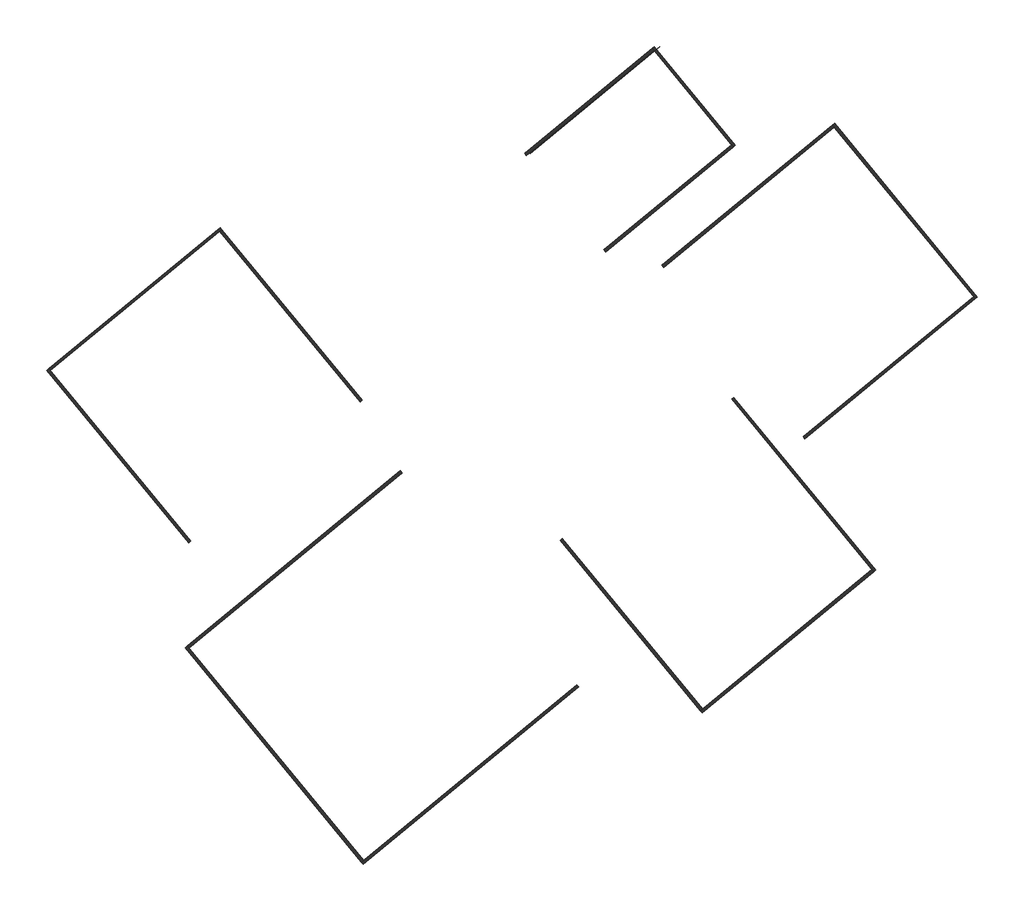
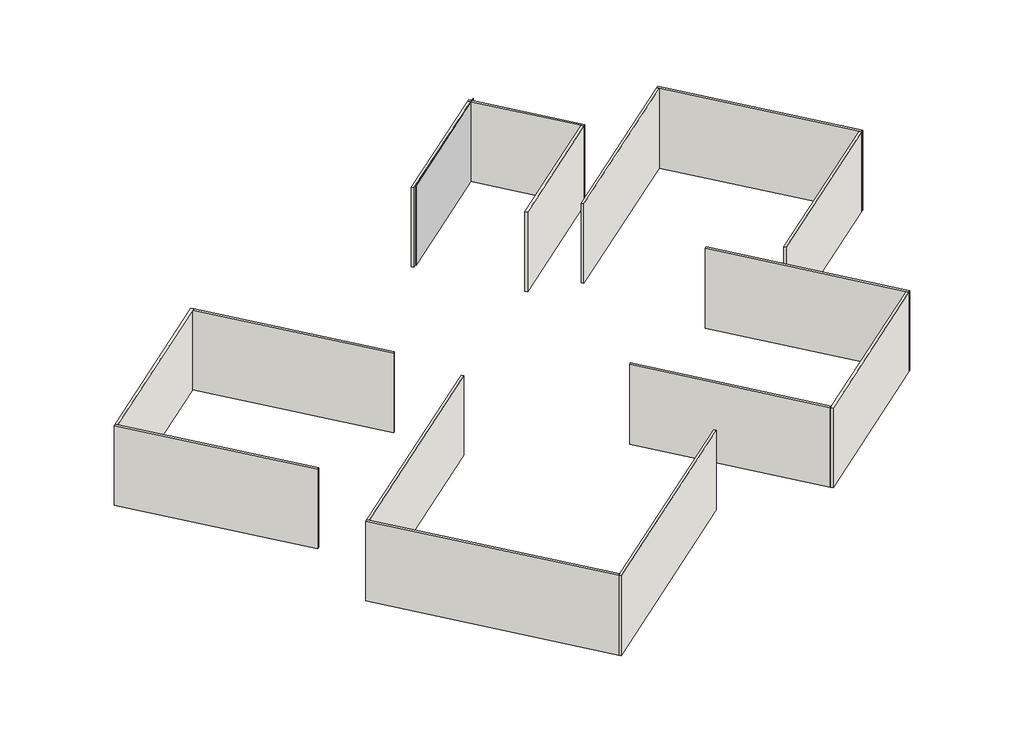
# One storey: 15 walls, 1 plate.
"""IFC4 building model written with IfcOpenShell, lengths in millimetres."""

import ifcopenshell
import ifcopenshell.guid

model = None  # the IFC model being written
_history = None  # IfcOwnerHistory: only IFC2X3 demands one
_inside = {}  # id of a spatial element -> (the spatial element, [elements in it])
_under = {}  # id of a project, library or spatial element -> (it, [spatial elements below it])
_declared = {}  # id of a project -> (the project, [libraries it declares])
_typed = {}  # id of a type object -> (the type object, [elements of that type])
_made_of = {}  # id of a material, layer set ... -> (it, [elements and type objects made of it])


def new_model(schema):
    """Start an empty IFC model of exactly this schema.

    Asked for "IFC4X3", IfcOpenShell would pick the latest addendum, in which some entities
    have other attributes; the version numbers below select the first issue.
    IFC2X3 requires an IfcOwnerHistory on every rooted entity: one is made here for all.
    """
    global model, _history
    if schema == "IFC4X3":
        model = ifcopenshell.file(schema_version=(4, 3, 0, 0))
    else:
        model = ifcopenshell.file(schema=schema)
    _inside.clear()
    _under.clear()
    _declared.clear()
    _typed.clear()
    _made_of.clear()
    _history = None
    if model.schema == "IFC2X3":
        org = make("IfcOrganization", Name="unknown")
        user = make(
            "IfcPersonAndOrganization",
            ThePerson=make("IfcPerson", FamilyName="unknown"),
            TheOrganization=org,
        )
        app = make(
            "IfcApplication",
            ApplicationDeveloper=org,
            Version="unknown",
            ApplicationFullName="unknown",
            ApplicationIdentifier="unknown",
        )
        _history = make(
            "IfcOwnerHistory",
            OwningUser=user,
            OwningApplication=app,
            ChangeAction="ADDED",
            CreationDate=0,
        )
    return model


def make(cls, **values):
    """One entity of the class cls with the attributes given. An attribute that is None is left unset."""
    return model.create_entity(
        cls, **{name: value for name, value in values.items() if value is not None}
    )


def rooted(cls, **values):
    """An entity with a GlobalId (a new one), such as an element, a storey or a relation."""
    return make(cls, GlobalId=ifcopenshell.guid.new(), OwnerHistory=_history, **values)


def si_unit(unit_type, name, prefix=None):
    """IfcSIUnit, for example si_unit("LENGTHUNIT", "METRE", prefix="MILLI")."""
    return make("IfcSIUnit", UnitType=unit_type, Prefix=prefix, Name=name)


def assignment(units):
    """IfcUnitAssignment: the units of a project."""
    return None if units is None else make("IfcUnitAssignment", Units=units)


def point(xyz):
    """IfcCartesianPoint."""
    return None if xyz is None else make("IfcCartesianPoint", Coordinates=xyz)


def direction(xyz):
    """IfcDirection."""
    return None if xyz is None else make("IfcDirection", DirectionRatios=xyz)


def frame(location, z_axis=None, x_axis=None):
    """IfcAxis2Placement3D, a coordinate frame: its origin and axes. An axis left out is left unset."""
    return make(
        "IfcAxis2Placement3D",
        Location=point(location),
        Axis=direction(z_axis),
        RefDirection=direction(x_axis),
    )


def origin():
    """The frame at (0, 0, 0) with its axes left unset."""
    return frame((0.0, 0.0, 0.0))


def origin_with_axes():
    """The frame at (0, 0, 0) with the z axis (0, 0, 1) and the x axis (1, 0, 0) written out."""
    return frame((0.0, 0.0, 0.0), z_axis=(0.0, 0.0, 1.0), x_axis=(1.0, 0.0, 0.0))


def place(relative_to, where):
    """IfcLocalPlacement: puts the frame where relative to a parent placement (None: the world)."""
    return make(
        "IfcLocalPlacement", PlacementRelTo=relative_to, RelativePlacement=where
    )


def context(
    kind, dimensions, precision=None, world=None, true_north=None, identifier=None
):
    """IfcGeometricRepresentationContext, for example the 3D "Model" context."""
    return make(
        "IfcGeometricRepresentationContext",
        ContextIdentifier=identifier,
        ContextType=kind,
        CoordinateSpaceDimension=dimensions,
        Precision=precision,
        WorldCoordinateSystem=world,
        TrueNorth=true_north,
    )


def project(units=None, contexts=None):
    """IfcProject with its units and contexts."""
    return rooted(
        "IfcProject",
        Name="project",
        RepresentationContexts=contexts,
        UnitsInContext=assignment(units),
    )


def spatial(cls, under=None, at=None, **own):
    """A site, building, storey or space (cls), placed at a placement, below another one or the project."""
    s = rooted(cls, ObjectPlacement=at, **own)
    if under is not None:
        _under.setdefault(under.id(), (under, []))[1].append(s)
    return s


def polyline(points):
    """IfcPolyline through the points."""
    return make("IfcPolyline", Points=[point(p) for p in points])


def outline(outer, holes=None, kind="AREA"):
    """IfcArbitraryClosedProfileDef: a profile drawn as a closed curve; with holes, ...WithVoids."""
    if holes is None:
        return make("IfcArbitraryClosedProfileDef", ProfileType=kind, OuterCurve=outer)
    return make(
        "IfcArbitraryProfileDefWithVoids",
        ProfileType=kind,
        OuterCurve=outer,
        InnerCurves=holes,
    )


def extrude(swept, where, along, depth):
    """IfcExtrudedAreaSolid: the profile swept, set in the frame where, extruded along a direction by depth."""
    return make(
        "IfcExtrudedAreaSolid",
        SweptArea=swept,
        Position=where,
        ExtrudedDirection=direction(along),
        Depth=depth,
    )


def faces_of(points, faces, orient=None, outer=None):
    """IfcFace entities. A face is a list of loops; a loop is a list of indices into points, from 0.

    orient and outer hold one flag for each loop. By default every Orientation is true, the
    first loop of a face is its IfcFaceOuterBound and the others are IfcFaceBound.
    """
    made = []
    for i, loops in enumerate(faces):
        bounds = []
        for j, loop in enumerate(loops):
            is_outer = j == 0 if outer is None else outer[i][j]
            bounds.append(
                make(
                    "IfcFaceOuterBound" if is_outer else "IfcFaceBound",
                    Bound=make("IfcPolyLoop", Polygon=[points[k] for k in loop]),
                    Orientation=True if orient is None else orient[i][j],
                )
            )
        made.append(make("IfcFace", Bounds=bounds))
    return made


def faceted_brep(points, faces, orient=None, outer=None, voids=None):
    """IfcFacetedBrep: a solid bounded by flat faces; with voids (closed shells), ...WithVoids."""
    shared = [point(p) for p in points]
    hull = make("IfcClosedShell", CfsFaces=faces_of(shared, faces, orient, outer))
    if voids is None:
        return make("IfcFacetedBrep", Outer=hull)
    return make(
        "IfcFacetedBrepWithVoids",
        Outer=hull,
        Voids=[
            make(cls, CfsFaces=faces_of(shared, fs, o, b)) for cls, fs, o, b in voids
        ],
    )


def shape(context_of_items, identifier, shape_type, items):
    """IfcShapeRepresentation: the items that make up one representation, for example the "Body"."""
    return make(
        "IfcShapeRepresentation",
        ContextOfItems=context_of_items,
        RepresentationIdentifier=identifier,
        RepresentationType=shape_type,
        Items=items,
    )


def source(mapping_origin, context_of_items, identifier, shape_type, items):
    """IfcRepresentationMap: a shape defined once, which mapped items show again and again."""
    return make(
        "IfcRepresentationMap",
        MappingOrigin=mapping_origin,
        MappedRepresentation=shape(context_of_items, identifier, shape_type, items),
    )


def transform(
    local_origin,
    x_axis=None,
    y_axis=None,
    z_axis=None,
    scale=None,
    scale2=None,
    scale3=None,
    uniform=True,
):
    """IfcCartesianTransformationOperator3D, or its non-uniform kind. x_axis, y_axis, z_axis: its Axis1, 2, 3."""
    if uniform:
        return make(
            "IfcCartesianTransformationOperator3D",
            Axis1=direction(x_axis),
            Axis2=direction(y_axis),
            LocalOrigin=point(local_origin),
            Scale=scale,
            Axis3=direction(z_axis),
        )
    return make(
        "IfcCartesianTransformationOperator3DnonUniform",
        Axis1=direction(x_axis),
        Axis2=direction(y_axis),
        LocalOrigin=point(local_origin),
        Scale=scale,
        Axis3=direction(z_axis),
        Scale2=scale2,
        Scale3=scale3,
    )


def mapped(mapping_source, mapping_target):
    """IfcMappedItem: shows the shape of a source again, moved by a transform."""
    return make(
        "IfcMappedItem", MappingSource=mapping_source, MappingTarget=mapping_target
    )


def made_of(thing, what):
    """Note that an element or type object is made of a material, layer set ...; save() writes the relation."""
    if what is not None:
        _made_of.setdefault(what.id(), (what, []))[1].append(thing)
    return thing


def element(
    cls,
    number,
    at=None,
    inside=None,
    cuts=None,
    type_object=None,
    material=None,
    context=None,
    identifier="Body",
    shape_type=None,
    held_by="IfcProductDefinitionShape",
    body=None,
    shapes=None,
    **own,
):
    """One element of the class cls, such as IfcWall. Its Tag is "e" and its number.

    at: its placement. inside: the storey or other place that contains it. cuts: it is an
    opening in that element (IfcRelVoidsElement). A single representation is given by context,
    identifier, shape_type and body (its items); several are given by shapes. held_by: the class
    of the entity that holds the representations. save() writes the other relations.
    """
    e = rooted(cls, Tag="e%d" % number, ObjectPlacement=at, **own)
    if body is not None:
        shapes = [shape(context, identifier, shape_type, body)]
    if shapes is not None:
        e.Representation = make(held_by, Representations=shapes)
    if inside is not None:
        _inside.setdefault(inside.id(), (inside, []))[1].append(e)
    if cuts is not None:
        rooted(
            "IfcRelVoidsElement", RelatingBuildingElement=cuts, RelatedOpeningElement=e
        )
    if type_object is not None:
        _typed.setdefault(type_object.id(), (type_object, []))[1].append(e)
    return made_of(e, material)


def aggregate(whole, parts):
    """IfcRelAggregates: a whole, such as a stair, and the parts it consists of."""
    return rooted("IfcRelAggregates", RelatingObject=whole, RelatedObjects=parts)


def save(model, path):
    """Write the relations noted so far, then the file.

    IfcRelAggregates (storeys below a building ...), IfcRelContainedInSpatialStructure (elements
    in a storey), IfcRelDefinesByType, IfcRelAssociatesMaterial and IfcRelDeclares: one each for
    every whole, place, type object, material and project.
    """
    for whole, parts in _under.values():
        aggregate(whole, parts)
    for where, things in _inside.values():
        rooted(
            "IfcRelContainedInSpatialStructure",
            RelatedElements=things,
            RelatingStructure=where,
        )
    for kind, things in _typed.values():
        rooted("IfcRelDefinesByType", RelatedObjects=things, RelatingType=kind)
    for what, things in _made_of.values():
        rooted("IfcRelAssociatesMaterial", RelatedObjects=things, RelatingMaterial=what)
    for by, libraries in _declared.values():
        rooted("IfcRelDeclares", RelatingContext=by, RelatedDefinitions=libraries)
    model.write(path)


def plate_433a51a3(model_context):
    return source(origin(), model_context, "Body", "SweptSolid", [
        extrude(outline(polyline([(6050.0, -12.5), (-6050.0, -12.5), (-6050.0, 12.5), (6050.0, 12.5), (6050.0, -12.5)])), origin_with_axes(), (0.0, 0.0, 1.0), 7200.0),
    ])


model = new_model("IFC4")

# Units and contexts
model_context = context("Model", 3, world=origin())
ifc_project = project(units=[si_unit("LENGTHUNIT", "METRE", prefix="MILLI")], contexts=[model_context])

# Site, building, storey
site = spatial("IfcSite", under=ifc_project)
building = spatial("IfcBuilding", under=site)
storey = spatial("IfcBuildingStorey", under=building, Name="f2-展厅", Elevation=10300.0)

# Plate
placement = place(None, origin())
plate_shape = plate_433a51a3(model_context)
element("IfcPlate", 1, ObjectType="系统嵌板 : 玻璃", at=placement, inside=storey, context=model_context, shape_type="MappedRepresentation", body=[
    mapped(plate_shape, transform((-12967.8381531, 29780.0656572, 10300.0), x_axis=(-0.7721557982734171, -0.6354332562848297, 0.0), y_axis=(0.6354332562848297, -0.7721557982734171, 0.0), z_axis=(0.0, 0.0, 1.0))),
])

# Walls
element("IfcWall", 2, ObjectType="aa-涂料-蓝色 - 200mm", at=placement, inside=storey, context=model_context, shape_type="Brep", body=[
    faceted_brep([(-29665.2352749, -25307.8357107, 10300.0), (-14144.9037296, -12535.6272594, 10300.0), (-14144.9037296, -12535.6272594, 17500.0), (-29665.2352749, -25307.8357107, 17500.0), (-29792.3219261, -25153.4045511, 10300.0), (-29792.3219261, -25153.4045511, 17500.0), (-29637.8907665, -25026.3178998, 17500.0), (-14271.9903808, -12381.1960997, 17500.0), (-14271.9903808, -12381.1960997, 10300.0), (-29637.8907665, -25026.3178998, 10300.0)], [[[0, 1, 2, 3]], [[4, 5, 6, 7, 8, 9]], [[1, 0, 4, 9, 8]], [[2, 1, 8, 7]], [[3, 2, 7, 6, 5]], [[0, 3, 5, 4]]]),
])
element("IfcWall", 3, ObjectType="aa-涂料-蓝色 - 200mm", at=placement, inside=storey, context=model_context, shape_type="Brep", body=[
    faceted_brep([(-42500.9870518, -9710.2885856, 10300.0), (-29792.3219261, -25153.4045511, 10300.0), (-29792.3219261, -25153.4045511, 17500.0), (-42500.9870518, -9710.2885856, 17500.0), (-42346.5558922, -9583.2019343, 10300.0), (-42346.5558922, -9583.2019343, 17500.0), (-42219.4692409, -9737.633094, 17500.0), (-29637.8907665, -25026.3178998, 17500.0), (-29637.8907665, -25026.3178998, 10300.0), (-42219.4692409, -9737.633094, 10300.0)], [[[0, 1, 2, 3]], [[4, 5, 6, 7, 8, 9]], [[1, 0, 4, 9, 8]], [[3, 2, 7, 6, 5]], [[2, 1, 8, 7]], [[0, 3, 5, 4]]]),
])
element("IfcWall", 4, ObjectType="aa-涂料-蓝色 - 200mm", at=placement, inside=storey, context=model_context, shape_type="SweptSolid", body=[
    extrude(outline(polyline([(-42346.5558922, -9583.2019343), (-26980.6555065, 3061.9198657), (-26853.5688553, 2907.4887061), (-42219.4692409, -9737.633094), (-42346.5558922, -9583.2019343)])), frame((0.0, 0.0, 10300.0), z_axis=(0.0, 0.0, 1.0), x_axis=(1.0, 0.0, 0.0)), (0.0, 0.0, 1.0), 7200.0),
])
element("IfcWall", 5, ObjectType="aa-涂料-蓝色 - 200mm", at=placement, inside=storey, context=model_context, shape_type="Brep", body=[
    faceted_brep([(-52476.6672312, 10289.7517826, 10300.0), (-42246.191805, -2141.9565696, 10300.0), (-42246.191805, -2141.9565696, 17500.0), (-52476.6672312, 10289.7517826, 17500.0), (-52322.2360716, 10416.8384338, 10300.0), (-52322.2360716, 10416.8384338, 17500.0), (-52195.1494203, 10262.4072742, 17500.0), (-42091.7606454, -2014.8699184, 17500.0), (-42091.7606454, -2014.8699184, 10300.0), (-52195.1494203, 10262.4072742, 10300.0)], [[[0, 1, 2, 3]], [[4, 5, 6, 7, 8, 9]], [[1, 0, 4, 9, 8]], [[2, 1, 8, 7]], [[3, 2, 7, 6, 5]], [[0, 3, 5, 4]]]),
])
element("IfcWall", 6, ObjectType="aa-涂料-蓝色 - 200mm", at=placement, inside=storey, context=model_context, shape_type="Brep", body=[
    faceted_brep([(-39967.7432992, 20583.7705344, 10300.0), (-52322.2360716, 10416.8384338, 10300.0), (-52322.2360716, 10416.8384338, 17500.0), (-39967.7432992, 20583.7705344, 17500.0), (-39840.6566479, 20429.3393747, 10300.0), (-39840.6566479, 20429.3393747, 17500.0), (-39995.0878076, 20302.2527235, 17500.0), (-52195.1494203, 10262.4072742, 17500.0), (-52195.1494203, 10262.4072742, 10300.0), (-39995.0878076, 20302.2527235, 10300.0)], [[[0, 1, 2, 3]], [[4, 5, 6, 7, 8, 9]], [[1, 0, 4, 9, 8]], [[3, 2, 7, 6, 5]], [[2, 1, 8, 7]], [[0, 3, 5, 4]]]),
])
element("IfcWall", 7, ObjectType="aa-涂料-蓝色 - 200mm", at=placement, inside=storey, context=model_context, shape_type="Brep", body=[
    faceted_brep([(14586.0882688, 15583.2088217, 10300.0), (4292.069517, 28092.1327537, 10300.0), (4292.069517, 28092.1327537, 17500.0), (14586.0882688, 15583.2088217, 17500.0), (14431.6571092, 15456.1221704, 10300.0), (14431.6571092, 15456.1221704, 17500.0), (14304.5704579, 15610.5533301, 17500.0), (4264.7250086, 27810.6149428, 17500.0), (4137.6383573, 27965.0461024, 17500.0), (4137.6383573, 27965.0461024, 10300.0), (4264.7250086, 27810.6149428, 10300.0), (14304.5704579, 15610.5533301, 10300.0)], [[[0, 1, 2, 3]], [[4, 5, 6, 7, 8, 9, 10, 11]], [[1, 0, 4, 11, 10, 9]], [[3, 2, 8, 7, 6, 5]], [[2, 1, 9, 8]], [[0, 3, 5, 4]]]),
])
element("IfcWall", 8, ObjectType="aa-涂料-蓝色 - 200mm", at=placement, inside=storey, context=model_context, shape_type="SweptSolid", body=[
    extrude(outline(polyline([(-8139.6388352, 17861.6573275), (4137.6383573, 27965.0461024), (4264.7250086, 27810.6149428), (-8012.5521839, 17707.2261679), (-8139.6388352, 17861.6573275)])), frame((0.0, 0.0, 10300.0), z_axis=(0.0, 0.0, 1.0), x_axis=(1.0, 0.0, 0.0)), (0.0, 0.0, 1.0), 7200.0),
])
element("IfcWall", 9, ObjectType="aa-涂料-蓝色 - 200mm", at=placement, inside=storey, context=model_context, shape_type="Brep", body=[
    faceted_brep([(-2850.3096158, 26520.6035137, 10300.0), (-8696.2955736, 33624.4368578, 10300.0), (-8696.2955736, 33624.4368578, 17500.0), (-2850.3096158, 26520.6035137, 17500.0), (-3004.7407754, 26393.5168624, 10300.0), (-3004.7407754, 26393.5168624, 17500.0), (-3131.8274267, 26547.9480221, 17500.0), (-8723.640082, 33342.9190469, 17500.0), (-8850.7267332, 33497.3502065, 17500.0), (-8850.7267332, 33497.3502065, 10300.0), (-8723.640082, 33342.9190469, 10300.0), (-3131.8274267, 26547.9480221, 10300.0)], [[[0, 1, 2, 3]], [[4, 5, 6, 7, 8, 9, 10, 11]], [[1, 0, 4, 11, 10, 9]], [[3, 2, 8, 7, 6, 5]], [[2, 1, 9, 8]], [[0, 3, 5, 4]]]),
])
element("IfcWall", 10, ObjectType="aa-涂料-蓝色 - 200mm", at=placement, inside=storey, context=model_context, shape_type="SweptSolid", body=[
    extrude(outline(polyline([(-18039.3807327, 25935.6944567), (-8850.7267332, 33497.3502065), (-8723.640082, 33342.9190469), (-17912.2940814, 25781.2632971), (-18039.3807327, 25935.6944567)])), frame((0.0, 0.0, 10300.0), z_axis=(0.0, 0.0, 1.0), x_axis=(1.0, 0.0, 0.0)), (0.0, 0.0, 1.0), 7200.0),
])
element("IfcWall", 11, ObjectType="aa-涂料-蓝色 - 200mm", at=placement, inside=storey, context=model_context, shape_type="SweptSolid", body=[
    extrude(outline(polyline([(-3004.7407754, 26393.5168624), (-12193.3947749, 18831.8611126), (-12320.4814261, 18986.2922723), (-3131.8274267, 26547.9480221), (-3004.7407754, 26393.5168624)])), frame((0.0, 0.0, 10300.0), z_axis=(0.0, 0.0, 1.0), x_axis=(1.0, 0.0, 0.0)), (0.0, 0.0, 1.0), 7200.0),
])
element("IfcWall", 12, ObjectType="aa-涂料-蓝色 - 200mm", at=placement, inside=storey, context=model_context, shape_type="SweptSolid", body=[
    extrude(outline(polyline([(14431.6571092, 15456.1221704), (2154.3799166, 5352.7333955), (2027.2932654, 5507.1645551), (14304.5704579, 15610.5533301), (14431.6571092, 15456.1221704)])), frame((0.0, 0.0, 10300.0), z_axis=(0.0, 0.0, 1.0), x_axis=(1.0, 0.0, 0.0)), (0.0, 0.0, 1.0), 7200.0),
])
element("IfcWall", 13, ObjectType="aa-涂料-蓝色 - 200mm", at=placement, inside=storey, context=model_context, shape_type="Brep", body=[
    faceted_brep([(7266.7909344, -4097.1139007, 10300.0), (-2963.6844918, 8334.5944515, 10300.0), (-2963.6844918, 8334.5944515, 17500.0), (7266.7909344, -4097.1139007, 17500.0), (7112.3597747, -4224.200552, 10300.0), (7112.3597747, -4224.200552, 17500.0), (6985.2731234, -4069.7693923, 17500.0), (-3118.1156515, 8207.5078003, 17500.0), (-3118.1156515, 8207.5078003, 10300.0), (6985.2731234, -4069.7693923, 10300.0)], [[[0, 1, 2, 3]], [[4, 5, 6, 7, 8, 9]], [[1, 0, 4, 9, 8]], [[2, 1, 8, 7]], [[3, 2, 7, 6, 5]], [[0, 3, 5, 4]]]),
])
element("IfcWall", 14, ObjectType="aa-涂料-蓝色 - 200mm", at=placement, inside=storey, context=model_context, shape_type="Brep", body=[
    faceted_brep([(-5242.1329977, -14391.1326525, 10300.0), (7112.3597747, -4224.200552, 10300.0), (7112.3597747, -4224.200552, 17500.0), (-5242.1329977, -14391.1326525, 17500.0), (-5369.2196489, -14236.7014929, 10300.0), (-5369.2196489, -14236.7014929, 17500.0), (-5214.7884893, -14109.6148416, 17500.0), (6985.2731234, -4069.7693923, 17500.0), (6985.2731234, -4069.7693923, 10300.0), (-5214.7884893, -14109.6148416, 10300.0)], [[[0, 1, 2, 3]], [[4, 5, 6, 7, 8, 9]], [[1, 0, 4, 9, 8]], [[3, 2, 7, 6, 5]], [[2, 1, 8, 7]], [[0, 3, 5, 4]]]),
])
element("IfcWall", 15, ObjectType="aa-涂料-蓝色 - 200mm", at=placement, inside=storey, context=model_context, shape_type="SweptSolid", body=[
    extrude(outline(polyline([(-5369.2196489, -14236.7014929), (-15472.6084239, -1959.4243003), (-15318.1772642, -1832.337649), (-5214.7884893, -14109.6148416), (-5369.2196489, -14236.7014929)])), frame((0.0, 0.0, 10300.0), z_axis=(0.0, 0.0, 1.0), x_axis=(1.0, 0.0, 0.0)), (0.0, 0.0, 1.0), 7200.0),
])
element("IfcWall", 16, ObjectType="aa-涂料-蓝色 - 200mm", at=placement, inside=storey, context=model_context, shape_type="SweptSolid", body=[
    extrude(outline(polyline([(-39840.6566479, 20429.3393747), (-29737.267873, 8152.0621822), (-29891.6990327, 8024.9755309), (-39995.0878076, 20302.2527235), (-39840.6566479, 20429.3393747)])), frame((0.0, 0.0, 10300.0), z_axis=(0.0, 0.0, 1.0), x_axis=(1.0, 0.0, 0.0)), (0.0, 0.0, 1.0), 7200.0),
])

save(model, "model.ifc")

# Revit data of these elements
# Type "系统嵌板 : 玻璃"
#   Construction Type Id = "GSP4R"
#   Analytic Construction = "1/8 英寸 Pilkington 单层玻璃"
#   Visual Light Transmittance = 0.9
#   Solar Heat Gain Coefficient = 0.86
#   Heat Transfer Coefficient (U) = 6.7069 W/(m²·K)
# Type "aa-涂料-蓝色 - 200mm"
#   Width = 200 mm
#   Layers, outside or top first: 200 mm "aa-涂料-蓝色" (function 1)
# Element 1 (IfcPlate, "系统嵌板 : 玻璃")
#   Phase Created = 新构造
#   Materials on its faces: "玻璃"
# Elements 2, 3, 4, 5, 6, 7, 8, 9, 10, 11, 12, 13, 14, 15, 16 (IfcWall, "aa-涂料-蓝色 - 200mm")
#   Top Offset = 0 mm
#   Base Offset = 0 mm
#   wall height = 7200 mm
#   Phase Created = 新构造
#   Base Constraint = f2-展厅
#   Top Constraint = f3-展厅
#   Materials on its faces: "aa-涂料-蓝色"
# Materials
#   "aa-涂料-蓝色": class "油漆", colour RGB 0 0 255, transparency 0
#   "玻璃": class "玻璃", colour RGB 0 128 192, transparency 0.9, Description = "钠钙玻璃", Cost = 0
